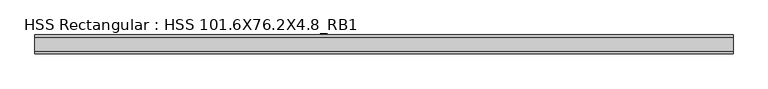
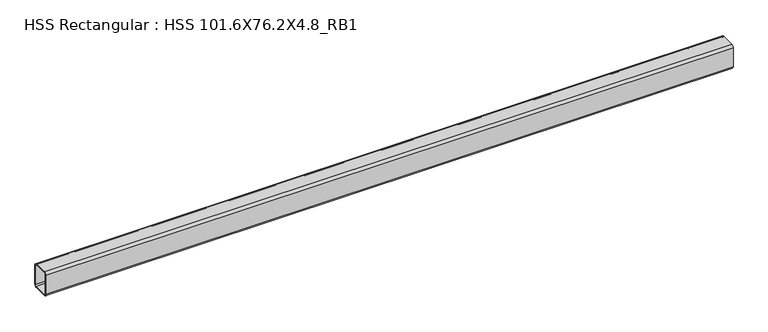
"""IFC4 building model written with IfcOpenShell, lengths in millimetres: beam geometry, HSS Rectangular : HSS 101.6X76.2X4.8_RB1."""

from ifc_helpers import new_model, si_unit, point, frame, frame_2d, origin, place, context, project, spatial, polyline, circle_curve, trimmed, segment, composite_curve, outline, extrude, source, transform, mapped, element, save


def hss_rectangular_hss_101_6x76_2x4_8_rb1_1ce7335e(model_context):
    return source(origin(), model_context, "Body", "SweptSolid", [
        extrude(outline(composite_curve([segment(polyline([(38.1, 41.275), (38.1, -41.275)]), True, "CONTINUOUS"), segment(trimmed(circle_curve(frame_2d((28.575, -41.275)), 9.525), [point((38.1, -41.275))], [point((28.575, -50.8))], False, "CARTESIAN"), True, "CONTINUOUS"), segment(polyline([(28.575, -50.8), (-28.575, -50.8)]), True, "CONTINUOUS"), segment(trimmed(circle_curve(frame_2d((-28.575, -41.275)), 9.525), [point((-28.575, -50.8))], [point((-38.1, -41.275))], False, "CARTESIAN"), True, "CONTINUOUS"), segment(polyline([(-38.1, -41.275), (-38.1, 41.275)]), True, "CONTINUOUS"), segment(trimmed(circle_curve(frame_2d((-28.575, 41.275)), 9.525), [point((-38.1, 41.275))], [point((-28.575, 50.8))], False, "CARTESIAN"), True, "CONTINUOUS"), segment(polyline([(-28.575, 50.8), (28.575, 50.8)]), True, "CONTINUOUS"), segment(trimmed(circle_curve(frame_2d((28.575, 41.275)), 9.525), [point((28.575, 50.8))], [point((38.1, 41.275))], False, "CARTESIAN"), True, "CONTINUOUS")], self_intersect=False), holes=[composite_curve([segment(trimmed(circle_curve(frame_2d((-28.575, 41.275)), 4.7625), [point((-28.575, 46.0375))], [point((-33.3375, 41.275))], True, "CARTESIAN"), True, "CONTINUOUS"), segment(polyline([(-33.3375, 41.275), (-33.3375, -41.275)]), True, "CONTINUOUS"), segment(trimmed(circle_curve(frame_2d((-28.575, -41.275)), 4.7625), [point((-33.3375, -41.275))], [point((-28.575, -46.0375))], True, "CARTESIAN"), True, "CONTINUOUS"), segment(polyline([(-28.575, -46.0375), (28.575, -46.0375)]), True, "CONTINUOUS"), segment(trimmed(circle_curve(frame_2d((28.575, -41.275)), 4.7625), [point((28.575, -46.0375))], [point((33.3375, -41.275))], True, "CARTESIAN"), True, "CONTINUOUS"), segment(polyline([(33.3375, -41.275), (33.3375, 41.275)]), True, "CONTINUOUS"), segment(trimmed(circle_curve(frame_2d((28.575, 41.275)), 4.7625), [point((33.3375, 41.275))], [point((28.575, 46.0375))], True, "CARTESIAN"), True, "CONTINUOUS"), segment(polyline([(28.575, 46.0375), (-28.575, 46.0375)]), True, "CONTINUOUS")], self_intersect=False)]), frame((-1410.625, 0.0, 0.0), z_axis=(1.0, 0.0, 0.0), x_axis=(0.0, 1.0, 0.0)), (0.0, 0.0, 1.0), 2821.25),
    ])


if __name__ == "__main__":
    model = new_model("IFC4")
    model_context = context("Model", 3, world=origin())
    ifc_project = project(units=[si_unit("LENGTHUNIT", "METRE", prefix="MILLI")], contexts=[model_context])
    site = spatial("IfcSite", under=ifc_project)
    building = spatial("IfcBuilding", under=site)
    placement = place(None, origin())
    hss_rectangular_hss_101_6x76_2x4_8_rb1_shape = hss_rectangular_hss_101_6x76_2x4_8_rb1_1ce7335e(model_context)
    element("IfcBeam", 1, ObjectType="HSS Rectangular : HSS 101.6X76.2X4.8_RB1", at=placement, inside=building, context=model_context, shape_type="MappedRepresentation", body=[
        mapped(hss_rectangular_hss_101_6x76_2x4_8_rb1_shape, transform((0.0, 0.0, 0.0), x_axis=(1.0, 0.0, 0.0), y_axis=(0.0, 1.0, 0.0), z_axis=(0.0, 0.0, 1.0))),
    ])
    save(model, "model.ifc")

# Revit data of these elements
# Type "HSS Rectangular : HSS 101.6X76.2X4.8_RB1"
#   Section Name Key = "HSS 4X3X3/16"
#   Assembly Code = "B10"
#   Width = 7.62 cm
#   Wall Nominal Thickness = 0.4763 cm
#   Wall Design Thickness = 0.442 cm
#   Torsional Moment of Inertia = 260.561 cm⁴
#   Torsional Modulus = 61.2876 cm³
#   Section Area = 14.4516 cm²
#   Plastic Modulus weak axis = 40.3122 cm³
#   Plastic Modulus strong axis = 49.1612 cm³
#   Perimeter = 0.881482 m²/m
#   Outer Fillet = 0.9525 cm
#   Nominal Weight = 12.1285 kgf/m
#   Moment of Inertia weak axis = 131.529 cm⁴
#   Moment of Inertia strong axis = 205.202 cm⁴
#   Inner Fillet = 0.4763 cm
#   Height = 10.16 cm
#   Elastic Modulus weak axis = 34.4128 cm³
#   Elastic Modulus strong axis = 40.476 cm³
#   Centroid Vertical = 5.08 cm
#   Centroid Horizontal = 3.81 cm
#   Length [instance default] = 1524 mm
#   Structural Material [instance default] = Steel ASTM A500, Grade B, Rectangular and Square
#   Principal Axes Angle = 0
# Element 1 (IfcBeam, "HSS Rectangular : HSS 101.6X76.2X4.8_RB1")
#   Structural Material = Steel ASTM A992
#   Materials on its faces: "Steel ASTM A992"
# Materials
#   "Steel ASTM A500, Grade B, Rectangular and Square": class "Metal", colour RGB 199 199 199, transparency 0, Description = "Carbon steel", Cost = 0
#   "Steel ASTM A992": class "Metal", colour RGB 199 199 199, transparency 0, Description = "Structural steel 50ksi", Cost = 0
